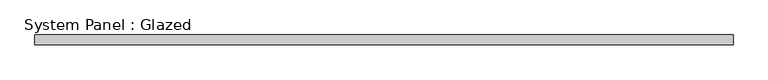
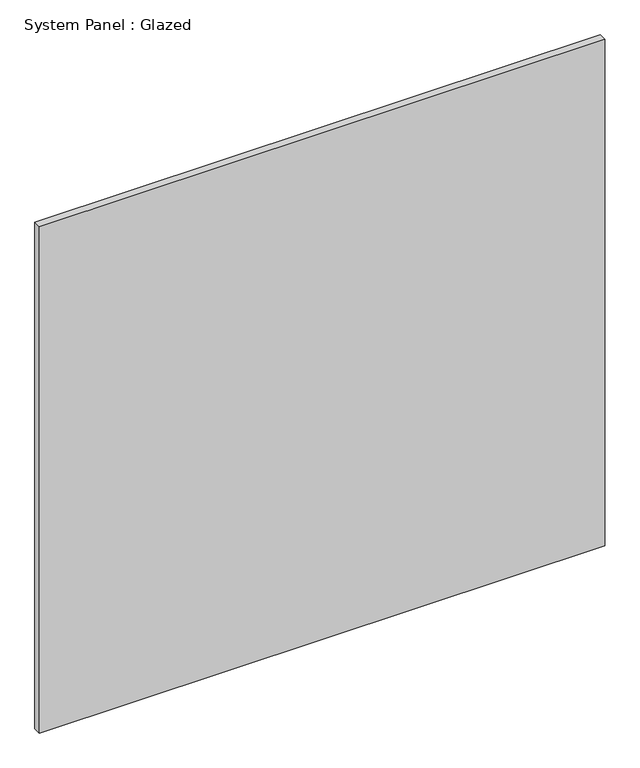
"""IFC4 building model written with IfcOpenShell, lengths in millimetres: plate geometry, System Panel : Glazed."""

from ifc_helpers import new_model, si_unit, origin, origin_with_axes, place, context, project, spatial, polyline, outline, extrude, source, transform, mapped, element, save


def system_panel_glazed_e1fe88a6(model_context):
    return source(origin(), model_context, "Body", "SweptSolid", [
        extrude(outline(polyline([(890.0, 24.5), (-890.0, 24.5), (-890.0, 49.5), (890.0, 49.5), (890.0, 24.5)])), origin_with_axes(), (0.0, 0.0, 1.0), 1686.2355347),
    ])


if __name__ == "__main__":
    model = new_model("IFC4")
    model_context = context("Model", 3, world=origin())
    ifc_project = project(units=[si_unit("LENGTHUNIT", "METRE", prefix="MILLI")], contexts=[model_context])
    site = spatial("IfcSite", under=ifc_project)
    building = spatial("IfcBuilding", under=site)
    placement = place(None, origin())
    system_panel_glazed_shape = system_panel_glazed_e1fe88a6(model_context)
    element("IfcPlate", 1, ObjectType="System Panel : Glazed", at=placement, inside=building, context=model_context, shape_type="MappedRepresentation", body=[
        mapped(system_panel_glazed_shape, transform((0.0, 0.0, 0.0), x_axis=(1.0, 0.0, 0.0), y_axis=(0.0, 1.0, 0.0), z_axis=(0.0, 0.0, 1.0))),
    ])
    save(model, "model.ifc")

# Revit data of these elements
# Element 1 (IfcPlate, "System Panel : Glazed")
#   Materials on its faces: "Glass"
# Materials
#   "Glass": class "Glass", colour RGB 218 227 224, transparency 0.85, Description = "Soda Lime Glass", Cost = 0
